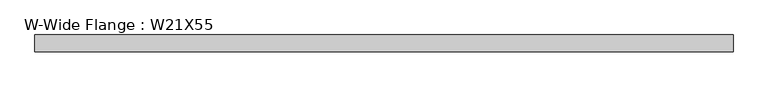
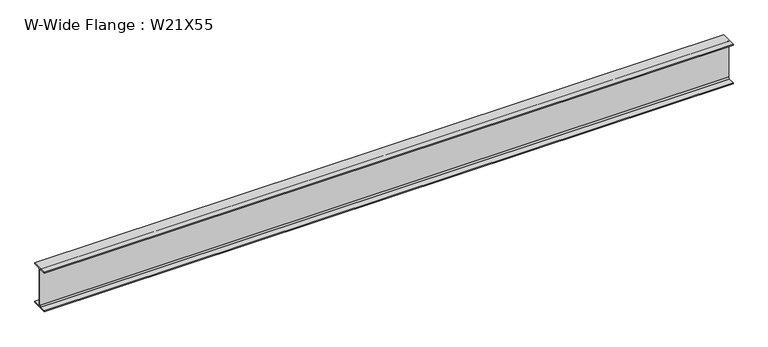
"""IFC4 building model written with IfcOpenShell, lengths in millimetres: beam geometry, W-Wide Flange : W21X55."""

from ifc_helpers import new_model, si_unit, point, frame, frame_2d, origin, place, context, project, spatial, polyline, circle_curve, trimmed, segment, composite_curve, outline, extrude, source, transform, mapped, element, save


def w_wide_flange_w21x55_01b98766(model_context):
    return source(origin(), model_context, "Body", "SweptSolid", [
        extrude(outline(composite_curve([segment(polyline([(104.394, -250.9012), (104.394, -264.16), (-104.394, -264.16), (-104.394, -250.9012), (-21.6662, -250.9012)]), True, "CONTINUOUS"), segment(trimmed(circle_curve(frame_2d((-21.6662, -233.9975)), 16.9037), [point((-21.6662, -250.9012))], [point((-4.7625, -233.9975))], True, "CARTESIAN"), True, "CONTINUOUS"), segment(polyline([(-4.7625, -233.9975), (-4.7625, 233.9975)]), True, "CONTINUOUS"), segment(trimmed(circle_curve(frame_2d((-21.6662, 233.9975)), 16.9037), [point((-4.7625, 233.9975))], [point((-21.6662, 250.9012))], True, "CARTESIAN"), True, "CONTINUOUS"), segment(polyline([(-21.6662, 250.9012), (-104.394, 250.9012), (-104.394, 264.16), (104.394, 264.16), (104.394, 250.9012), (21.6662, 250.9012)]), True, "CONTINUOUS"), segment(trimmed(circle_curve(frame_2d((21.6662, 233.9975)), 16.9037), [point((21.6662, 250.9012))], [point((4.7625, 233.9975))], True, "CARTESIAN"), True, "CONTINUOUS"), segment(polyline([(4.7625, 233.9975), (4.7625, -233.9975)]), True, "CONTINUOUS"), segment(trimmed(circle_curve(frame_2d((21.6662, -233.9975)), 16.9037), [point((4.7625, -233.9975))], [point((21.6662, -250.9012))], True, "CARTESIAN"), True, "CONTINUOUS"), segment(polyline([(21.6662, -250.9012), (104.394, -250.9012)]), True, "CONTINUOUS")], self_intersect=False)), frame((-4368.8, 0.0, 0.0), z_axis=(1.0, 0.0, 0.0), x_axis=(0.0, 1.0, 0.0)), (0.0, 0.0, 1.0), 8737.6),
    ])


if __name__ == "__main__":
    model = new_model("IFC4")
    model_context = context("Model", 3, world=origin())
    ifc_project = project(units=[si_unit("LENGTHUNIT", "METRE", prefix="MILLI")], contexts=[model_context])
    site = spatial("IfcSite", under=ifc_project)
    building = spatial("IfcBuilding", under=site)
    placement = place(None, origin())
    w_wide_flange_w21x55_shape = w_wide_flange_w21x55_01b98766(model_context)
    element("IfcBeam", 1, ObjectType="W-Wide Flange : W21X55", at=placement, inside=building, context=model_context, shape_type="MappedRepresentation", body=[
        mapped(w_wide_flange_w21x55_shape, transform((0.0, 0.0, 0.0), x_axis=(1.0, 0.0, 0.0), y_axis=(0.0, 1.0, 0.0), z_axis=(0.0, 0.0, 1.0))),
    ])
    save(model, "model.ifc")

# Revit data of these elements
# Type "W-Wide Flange : W21X55"
#   Assembly Code = "B10"
#   W = 55
#   Length [instance default] = 5' - 0"
#   bf = 0' - 8.22"
#   d = 1' - 8.8"
#   k = 0' - 1 3/16"
#   k2 = 0' - 0.6655"
#   tf = 0' - 0.522"
#   tw = 0' - 0 3/8"
#   A = 0.1125 SF
#   Structural Material [instance default] = Steel ASTM A992
# Element 1 (IfcBeam, "W-Wide Flange : W21X55")
#   Materials on its faces: "Steel ASTM A992"
# Materials
#   "Steel ASTM A992": class "Metal", colour RGB 199 199 199, transparency 0, Description = "Structural steel 50ksi", Cost = 0
